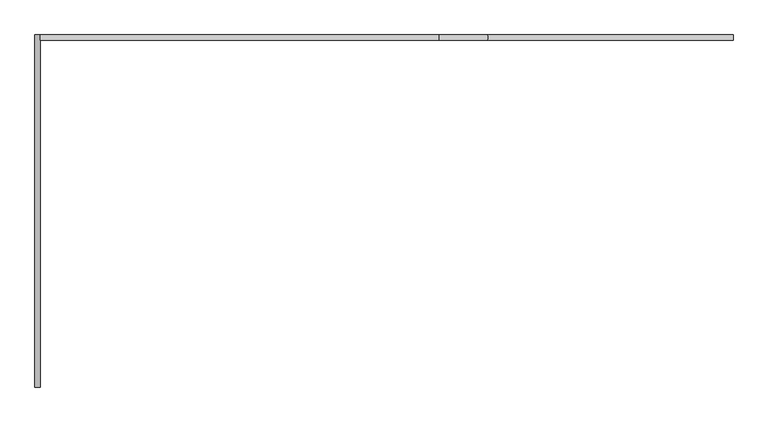
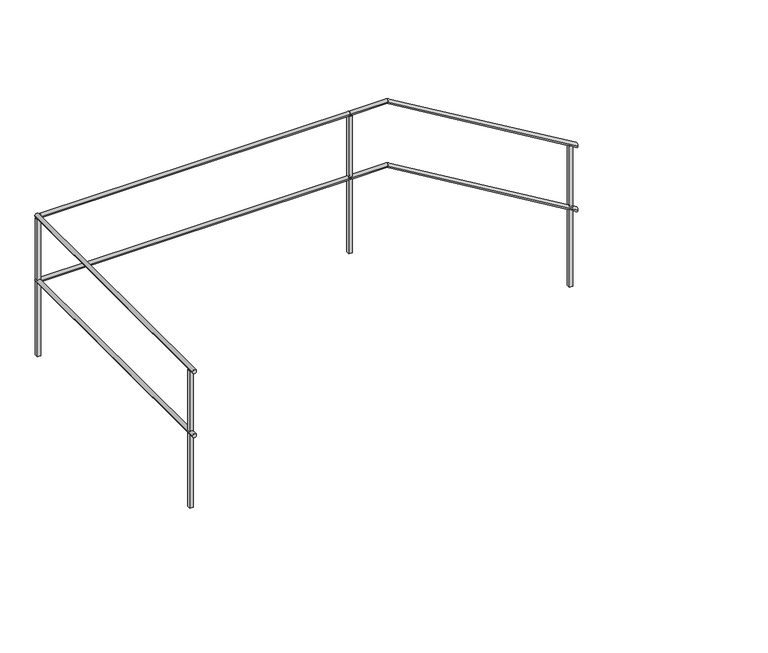
"""IFC4 building model written with IfcOpenShell, lengths in millimetres: railing geometry."""

from ifc_helpers import new_model, si_unit, frame, origin, place, context, project, spatial, polyline, circle_curve, ellipse_curve, outline, extrude, source, transform, mapped, element, save
from ifc_brep_helpers import plane_surface, cylinder_surface, advanced_brep


def railing_1d3e81d1(model_context):
    return source(origin(), model_context, "Body", "SolidModel", [
        advanced_brep(
        [(33043.8956602, 25734.1208589, 749.1723166), (33043.8956602, 25764.1208589, 749.1723166), (31639.7692216, 25734.1208589, 1584.9618634), (31639.7692216, 25764.1208589, 1584.9618634), (31363.8956602, 25734.1208589, 1584.9618634), (31363.8956602, 25764.1208589, 1584.9618634)],
        [
            (0, 1, ellipse_curve(frame((33043.8956602, 25749.1208589, 749.1723166), z_axis=(1.0, 0.0, 0.0), x_axis=(0.0, 0.0, -1.0)), 17.4562134, 15.0)),
            (1, 0, ellipse_curve(frame((33043.8956602, 25749.1208589, 749.1723166), z_axis=(1.0, 0.0, 0.0), x_axis=(0.0, 0.0, -1.0)), 17.4562134, 15.0)),
            (0, 2),
            (2, 3, ellipse_curve(frame((31639.7692216, 25749.1208589, 1584.9618634), z_axis=(0.9641817474962142, 0.0, -0.26524245096731175), x_axis=(-0.26524245096731197, 0.0, -0.964181747496214)), 15.5572329, 15.0)),
            (3, 1),
            (3, 2, ellipse_curve(frame((31639.7692216, 25749.1208589, 1584.9618634), z_axis=(0.9641817474962142, 0.0, -0.26524245096731175), x_axis=(-0.26524245096731197, 0.0, -0.964181747496214)), 15.5572329, 15.0)),
            (4, 5, circle_curve(frame((31363.8956602, 25749.1208589, 1584.9618634), z_axis=(-1.0, 0.0, 0.0), x_axis=(0.0, 1.0, 0.0)), 15.0)),
            (5, 4, circle_curve(frame((31363.8956602, 25749.1208589, 1584.9618634), z_axis=(-1.0, 0.0, 0.0), x_axis=(0.0, 1.0, 0.0)), 15.0)),
            (2, 4),
            (5, 3),
        ],
        [
            plane_surface(frame((33043.8956602, 25749.1208589, 766.62853), z_axis=(1.0, 0.0, 0.0), x_axis=(0.0, -1.0, 0.0))),
            cylinder_surface(frame((33036.2234023, 25749.1208589, 753.7391368), z_axis=(0.8592928844097065, 0.0, -0.5114838597676831), x_axis=(0.0, 1.0, 0.0)), 15.0),
            plane_surface(frame((31363.8956602, 25749.1208589, 1599.9618634), z_axis=(-1.0, 0.0, 0.0), x_axis=(0.0, -1.0, 0.0))),
            cylinder_surface(frame((31643.8956602, 25749.1208589, 1584.9618634), z_axis=(1.0, 0.0, 0.0), x_axis=(0.0, 1.0, 0.0)), 15.0),
        ],
        [
            (0, [[1, 2]]),
            (1, [[-1, 3, 4, 5]]),
            (1, [[-2, -5, 6, -3]]),
            (2, [[7, 8]]),
            (3, [[-4, 9, -8, 10]]),
            (3, [[-6, -10, -7, -9]]),
        ],
    ),
        advanced_brep(
        [(31363.8956602, 25734.1208589, 1584.9618634), (31363.8956602, 25764.1208589, 1584.9618634), (29079.2956602, 25734.1208589, 1584.9618634), (29079.2956602, 25764.1208589, 1584.9618634)],
        [
            (0, 1, circle_curve(frame((31363.8956602, 25749.1208589, 1584.9618634), z_axis=(1.0, 0.0, 0.0), x_axis=(0.0, 1.0, 0.0)), 15.0)),
            (1, 0, circle_curve(frame((31363.8956602, 25749.1208589, 1584.9618634), z_axis=(1.0, 0.0, 0.0), x_axis=(0.0, 1.0, 0.0)), 15.0)),
            (2, 3, circle_curve(frame((29079.2956602, 25749.1208589, 1584.9618634), z_axis=(-1.0, 0.0, 0.0), x_axis=(0.0, 1.0, 0.0)), 15.0)),
            (3, 2, circle_curve(frame((29079.2956602, 25749.1208589, 1584.9618634), z_axis=(-1.0, 0.0, 0.0), x_axis=(0.0, 1.0, 0.0)), 15.0)),
            (0, 2),
            (3, 1),
        ],
        [
            plane_surface(frame((31363.8956602, 25749.1208589, 1599.9618634), z_axis=(1.0, 0.0, 0.0), x_axis=(0.0, -1.0, 0.0))),
            plane_surface(frame((29079.2956602, 25749.1208589, 1599.9618634), z_axis=(-1.0, 0.0, 0.0), x_axis=(0.0, -1.0, 0.0))),
            cylinder_surface(frame((31363.8956602, 25749.1208589, 1584.9618634), z_axis=(1.0, 0.0, 0.0), x_axis=(0.0, 1.0, 0.0)), 15.0),
        ],
        [
            (0, [[1, 2]]),
            (1, [[3, 4]]),
            (2, [[-1, 5, -4, 6]]),
            (2, [[-2, -6, -3, -5]]),
        ],
    ),
        advanced_brep(
        [(29079.2956602, 25764.1208589, 1584.9618634), (29049.2956602, 25764.1208589, 1584.9618634), (29079.2956602, 23749.5208589, 1584.9618634), (29049.2956602, 23749.5208589, 1584.9618634)],
        [
            (0, 1, circle_curve(frame((29064.2956602, 25764.1208589, 1584.9618634), z_axis=(0.0, 1.0, 0.0), x_axis=(-1.0, 0.0, 0.0)), 15.0)),
            (1, 0, circle_curve(frame((29064.2956602, 25764.1208589, 1584.9618634), z_axis=(0.0, 1.0, 0.0), x_axis=(-1.0, 0.0, 0.0)), 15.0)),
            (2, 3, circle_curve(frame((29064.2956602, 23749.5208589, 1584.9618634), z_axis=(0.0, -1.0, 0.0), x_axis=(-1.0, 0.0, 0.0)), 15.0)),
            (3, 2, circle_curve(frame((29064.2956602, 23749.5208589, 1584.9618634), z_axis=(0.0, -1.0, 0.0), x_axis=(-1.0, 0.0, 0.0)), 15.0)),
            (0, 2),
            (3, 1),
        ],
        [
            plane_surface(frame((29064.2956602, 25764.1208589, 1599.9618634), z_axis=(0.0, 1.0, 0.0), x_axis=(0.0, 0.0, -1.0))),
            plane_surface(frame((29064.2956602, 23749.5208589, 1599.9618634), z_axis=(0.0, -1.0, 0.0), x_axis=(0.0, 0.0, -1.0))),
            cylinder_surface(frame((29064.2956602, 25764.1208589, 1584.9618634), z_axis=(0.0, 1.0, 0.0), x_axis=(-1.0, 0.0, 0.0)), 15.0),
        ],
        [
            (0, [[1, 2]]),
            (1, [[3, 4]]),
            (2, [[-1, 5, -4, 6]]),
            (2, [[-2, -6, -3, -5]]),
        ],
    ),
        advanced_brep(
        [(33043.8956602, 25734.1208589, 1249.1723166), (33043.8956602, 25764.1208589, 1249.1723166), (31639.7692216, 25734.1208589, 2084.9618634), (31639.7692216, 25764.1208589, 2084.9618634), (31363.8956602, 25734.1208589, 2084.9618634), (31363.8956602, 25764.1208589, 2084.9618634)],
        [
            (0, 1, ellipse_curve(frame((33043.8956602, 25749.1208589, 1249.1723166), z_axis=(1.0, 0.0, 0.0), x_axis=(0.0, 0.0, -1.0)), 17.4562134, 15.0)),
            (1, 0, ellipse_curve(frame((33043.8956602, 25749.1208589, 1249.1723166), z_axis=(1.0, 0.0, 0.0), x_axis=(0.0, 0.0, -1.0)), 17.4562134, 15.0)),
            (0, 2),
            (2, 3, ellipse_curve(frame((31639.7692216, 25749.1208589, 2084.9618634), z_axis=(0.9641817474962142, 0.0, -0.26524245096731175), x_axis=(-0.26524245096731197, 0.0, -0.964181747496214)), 15.5572329, 15.0)),
            (3, 1),
            (3, 2, ellipse_curve(frame((31639.7692216, 25749.1208589, 2084.9618634), z_axis=(0.9641817474962142, 0.0, -0.26524245096731175), x_axis=(-0.26524245096731197, 0.0, -0.964181747496214)), 15.5572329, 15.0)),
            (4, 5, circle_curve(frame((31363.8956602, 25749.1208589, 2084.9618634), z_axis=(-1.0, 0.0, 0.0), x_axis=(0.0, 1.0, 0.0)), 15.0)),
            (5, 4, circle_curve(frame((31363.8956602, 25749.1208589, 2084.9618634), z_axis=(-1.0, 0.0, 0.0), x_axis=(0.0, 1.0, 0.0)), 15.0)),
            (2, 4),
            (5, 3),
        ],
        [
            plane_surface(frame((33043.8956602, 25749.1208589, 1266.62853), z_axis=(1.0, 0.0, 0.0), x_axis=(0.0, -1.0, 0.0))),
            cylinder_surface(frame((33036.2234023, 25749.1208589, 1253.7391368), z_axis=(0.8592928844097065, 0.0, -0.5114838597676831), x_axis=(0.0, 1.0, 0.0)), 15.0),
            plane_surface(frame((31363.8956602, 25749.1208589, 2099.9618634), z_axis=(-1.0, 0.0, 0.0), x_axis=(0.0, -1.0, 0.0))),
            cylinder_surface(frame((31643.8956602, 25749.1208589, 2084.9618634), z_axis=(1.0, 0.0, 0.0), x_axis=(0.0, 1.0, 0.0)), 15.0),
        ],
        [
            (0, [[1, 2]]),
            (1, [[-1, 3, 4, 5]]),
            (1, [[-2, -5, 6, -3]]),
            (2, [[7, 8]]),
            (3, [[-4, 9, -8, 10]]),
            (3, [[-6, -10, -7, -9]]),
        ],
    ),
        advanced_brep(
        [(31363.8956602, 25734.1208589, 2084.9618634), (31363.8956602, 25764.1208589, 2084.9618634), (29079.2956602, 25734.1208589, 2084.9618634), (29079.2956602, 25764.1208589, 2084.9618634)],
        [
            (0, 1, circle_curve(frame((31363.8956602, 25749.1208589, 2084.9618634), z_axis=(1.0, 0.0, 0.0), x_axis=(0.0, 1.0, 0.0)), 15.0)),
            (1, 0, circle_curve(frame((31363.8956602, 25749.1208589, 2084.9618634), z_axis=(1.0, 0.0, 0.0), x_axis=(0.0, 1.0, 0.0)), 15.0)),
            (2, 3, circle_curve(frame((29079.2956602, 25749.1208589, 2084.9618634), z_axis=(-1.0, 0.0, 0.0), x_axis=(0.0, 1.0, 0.0)), 15.0)),
            (3, 2, circle_curve(frame((29079.2956602, 25749.1208589, 2084.9618634), z_axis=(-1.0, 0.0, 0.0), x_axis=(0.0, 1.0, 0.0)), 15.0)),
            (0, 2),
            (3, 1),
        ],
        [
            plane_surface(frame((31363.8956602, 25749.1208589, 2099.9618634), z_axis=(1.0, 0.0, 0.0), x_axis=(0.0, -1.0, 0.0))),
            plane_surface(frame((29079.2956602, 25749.1208589, 2099.9618634), z_axis=(-1.0, 0.0, 0.0), x_axis=(0.0, -1.0, 0.0))),
            cylinder_surface(frame((31363.8956602, 25749.1208589, 2084.9618634), z_axis=(1.0, 0.0, 0.0), x_axis=(0.0, 1.0, 0.0)), 15.0),
        ],
        [
            (0, [[1, 2]]),
            (1, [[3, 4]]),
            (2, [[-1, 5, -4, 6]]),
            (2, [[-2, -6, -3, -5]]),
        ],
    ),
        advanced_brep(
        [(29079.2956602, 25764.1208589, 2084.9618634), (29049.2956602, 25764.1208589, 2084.9618634), (29079.2956602, 23749.5208589, 2084.9618634), (29049.2956602, 23749.5208589, 2084.9618634)],
        [
            (0, 1, circle_curve(frame((29064.2956602, 25764.1208589, 2084.9618634), z_axis=(0.0, 1.0, 0.0), x_axis=(-1.0, 0.0, 0.0)), 15.0)),
            (1, 0, circle_curve(frame((29064.2956602, 25764.1208589, 2084.9618634), z_axis=(0.0, 1.0, 0.0), x_axis=(-1.0, 0.0, 0.0)), 15.0)),
            (2, 3, circle_curve(frame((29064.2956602, 23749.5208589, 2084.9618634), z_axis=(0.0, -1.0, 0.0), x_axis=(-1.0, 0.0, 0.0)), 15.0)),
            (3, 2, circle_curve(frame((29064.2956602, 23749.5208589, 2084.9618634), z_axis=(0.0, -1.0, 0.0), x_axis=(-1.0, 0.0, 0.0)), 15.0)),
            (0, 2),
            (3, 1),
        ],
        [
            plane_surface(frame((29064.2956602, 25764.1208589, 2099.9618634), z_axis=(0.0, 1.0, 0.0), x_axis=(0.0, 0.0, -1.0))),
            plane_surface(frame((29064.2956602, 23749.5208589, 2099.9618634), z_axis=(0.0, -1.0, 0.0), x_axis=(0.0, 0.0, -1.0))),
            cylinder_surface(frame((29064.2956602, 25764.1208589, 2084.9618634), z_axis=(0.0, 1.0, 0.0), x_axis=(-1.0, 0.0, 0.0)), 15.0),
        ],
        [
            (0, [[1, 2]]),
            (1, [[3, 4]]),
            (2, [[-1, 5, -4, 6]]),
            (2, [[-2, -6, -3, -5]]),
        ],
    ),
        extrude(outline(polyline([(29076.7956602, 25761.6208589), (29076.7956602, 25736.6208589), (29051.7956602, 25736.6208589), (29051.7956602, 25761.6208589), (29076.7956602, 25761.6208589)])), frame((0.0, 0.0, 999.9618634), z_axis=(0.0, 0.0, 1.0), x_axis=(1.0, 0.0, 0.0)), (0.0, 0.0, 1.0), 1070.0),
        extrude(outline(polyline([(31376.3956602, 25761.6208589), (31376.3956602, 25736.6208589), (31351.3956602, 25736.6208589), (31351.3956602, 25761.6208589), (31376.3956602, 25761.6208589)])), frame((0.0, 0.0, 999.9618634), z_axis=(0.0, 0.0, 1.0), x_axis=(1.0, 0.0, 0.0)), (0.0, 0.0, 1.0), 1070.0),
        extrude(outline(polyline([(29051.7956602, 23812.0208589), (29076.7956602, 23812.0208589), (29076.7956602, 23787.0208589), (29051.7956602, 23787.0208589), (29051.7956602, 23812.0208589)])), frame((0.0, 0.0, 999.9618634), z_axis=(0.0, 0.0, 1.0), x_axis=(1.0, 0.0, 0.0)), (0.0, 0.0, 1.0), 1070.0),
        extrude(outline(polyline([(166.62853, 33006.3956602), (1258.9499586, 33006.3956602), (1273.830911, 32981.3956602), (166.62853, 32981.3956602), (166.62853, 33006.3956602)])), frame((0.0, 25736.6208589, 0.0), z_axis=(0.0, 1.0, 0.0), x_axis=(0.0, 0.0, 1.0)), (0.0, 0.0, 1.0), 25.0),
    ])


if __name__ == "__main__":
    model = new_model("IFC4")
    model_context = context("Model", 3, world=origin())
    ifc_project = project(units=[si_unit("LENGTHUNIT", "METRE", prefix="MILLI")], contexts=[model_context])
    site = spatial("IfcSite", under=ifc_project)
    building = spatial("IfcBuilding", under=site)
    placement = place(None, origin())
    railing_shape = railing_1d3e81d1(model_context)
    element("IfcRailing", 1, at=placement, inside=building, context=model_context, shape_type="MappedRepresentation", body=[
        mapped(railing_shape, transform((0.0, 0.0, 0.0), x_axis=(1.0, 0.0, 0.0), y_axis=(0.0, 1.0, 0.0), z_axis=(0.0, 0.0, 1.0))),
    ])
    save(model, "model.ifc")
